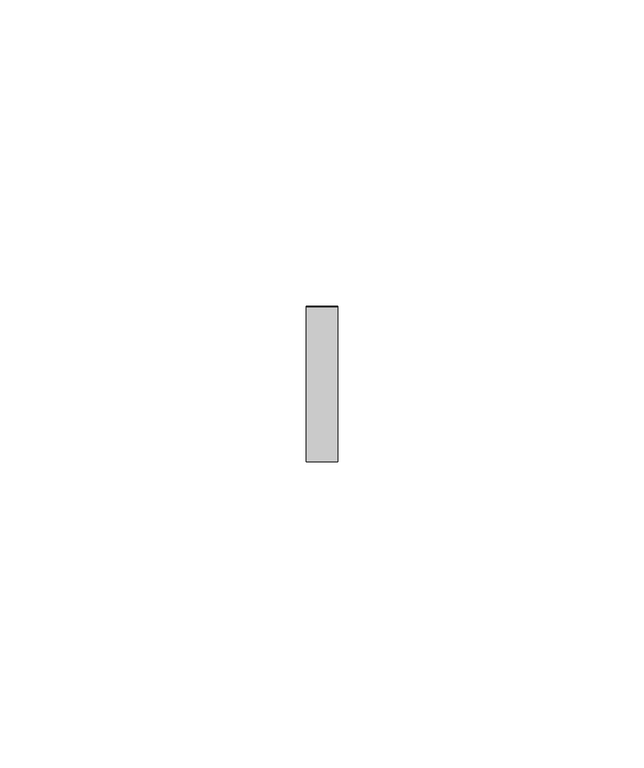
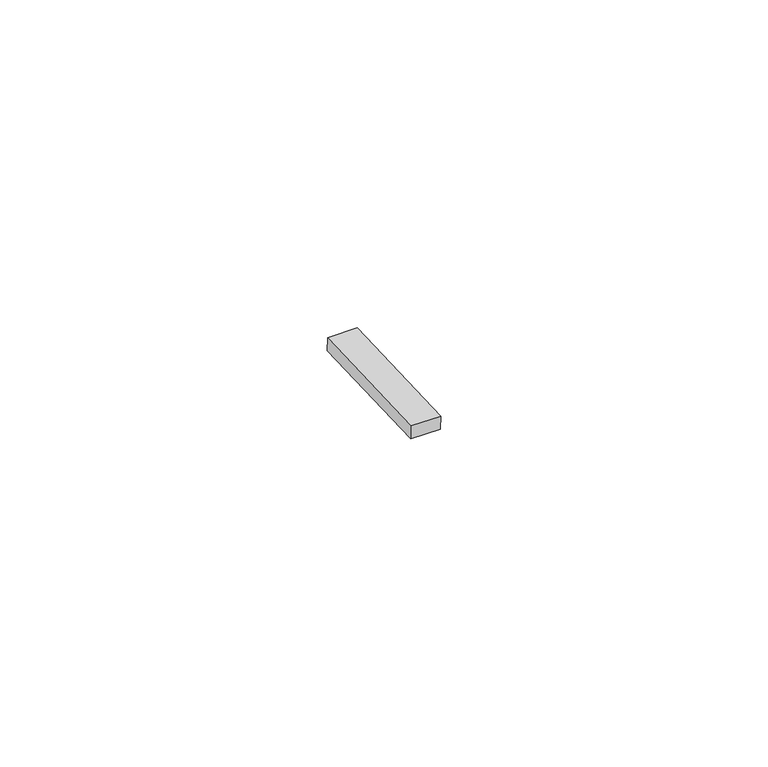
"""IFC4 building model written with IfcOpenShell, lengths in millimetres: proxy geometry, Inner panel:Inner panel:1:Inner panel:1 : Inner panel:Inner panel:300324:2:Inner panel:1:Inner panel:1 : Inner panel:Inner panel:300324:2 : Inner panel:Inner panel:1:Inner panel:1 : Inner panel:Inner panel:300324:300043:108 : Inner panel:Inner panel:1:Inner panel:1 : Inner panel:Inner panel:300324:2:Inner panel:1:Inner panel:1 : Inner panel:Inner panel:300324:2 : Inner panel:Inner panel:1:Inner panel:1 : Inner panel:Inner panel:300324:300043:308120."""

from ifc_helpers import new_model, si_unit, frame, origin, place, context, project, spatial, polyline, outline, extrude, source, transform, mapped, element, save


def generic_models_c30442cb(model_context):
    return source(origin(), model_context, "Body", "SweptSolid", [
        extrude(outline(polyline([(0.0, -25.4), (0.0, 0.0), (5.2138089, 0.0), (5.2138089, -25.4), (0.0, -25.4)])), frame((593530.195117, -576574.3073926, 4050.9976844), z_axis=(0.0, -0.041630544712223896, 0.9991330730923502), x_axis=(-1.0, 0.0, 0.0)), (0.0, 0.0, 1.0), 2.4763745),
    ])


if __name__ == "__main__":
    model = new_model("IFC4")
    model_context = context("Model", 3, world=origin())
    ifc_project = project(units=[si_unit("LENGTHUNIT", "METRE", prefix="MILLI")], contexts=[model_context])
    site = spatial("IfcSite", under=ifc_project)
    building = spatial("IfcBuilding", under=site)
    placement = place(None, origin())
    generic_models_shape = generic_models_c30442cb(model_context)
    element("IfcBuildingElementProxy", 1, Name="Inner panel:Inner panel:1:Inner panel:1 : Inner panel:Inner panel:300324:2:Inner panel:1:Inner panel:1 : Inner panel:Inner panel:300324:2 : Inner panel:Inner panel:1:Inner panel:1 : Inner panel:Inner panel:300324:300043:108 : Inner panel:Inner panel:1:Inner panel:1 : Inner panel:Inner panel:300324:2:Inner panel:1:Inner panel:1 : Inner panel:Inner panel:300324:2 : Inner panel:Inner panel:1:Inner panel:1 : Inner panel:Inner panel:300324:300043:308120", ObjectType="Inner panel:Inner panel:1:Inner panel:1 : Inner panel:Inner panel:300324:2:Inner panel:1:Inner panel:1 : Inner panel:Inner panel:300324:2 : Inner panel:Inner panel:1:Inner panel:1 : Inner panel:Inner panel:300324:300043:108 : Inner panel:Inner panel:1:Inner panel:1 : Inner panel:Inner panel:300324:2:Inner panel:1:Inner panel:1 : Inner panel:Inner panel:300324:2 : Inner panel:Inner panel:1:Inner panel:1 : Inner panel:Inner panel:300324:300043:308120", at=placement, inside=building, context=model_context, shape_type="MappedRepresentation", body=[
        mapped(generic_models_shape, transform((0.0, 0.0, 0.0), x_axis=(1.0, 0.0, 0.0), y_axis=(0.0, 1.0, 0.0), z_axis=(0.0, 0.0, 1.0))),
    ])
    save(model, "model.ifc")

# Revit data of these elements
# Type "Inner panel:Inner panel:1:Inner panel:1 : Inner panel:Inner panel:300324:2:Inner panel:1:Inner panel:1 : Inner panel:Inner panel:300324:2 : Inner panel:Inner panel:1:Inner panel:1 : Inner panel:Inner panel:300324:300043:108 : Inner panel:Inner panel:1:Inner panel:1 : Inner panel:Inner panel:300324:2:Inner panel:1:Inner panel:1 : Inner panel:Inner panel:300324:2 : Inner panel:Inner panel:1:Inner panel:1 : Inner panel:Inner panel:300324:300043:308120"
#   NameOverride = "Inner panel:Inner panel:1:Inner panel:1 : Inner panel:Inner panel:300324:2:Inner panel:1:Inner panel:1 : Inner panel:Inner panel:300324:2 : Inner panel:Inner panel:1:Inner panel:1 : Inner panel:Inner panel:300324:300043:308120"
#   ObjectTypeOverride = "Inner panel:1:Inner panel:1 : Inner panel:Inner panel:300324:2 : Inner panel:Inner panel:1:Inner panel:1 : Inner panel:Inner panel:300324:300043"
#   Reference = "Inner panel"
#   Tag = "308120"
# Element 1 (IfcBuildingElementProxy, "Inner panel:Inner panel:1:Inner panel:1 : Inner panel:Inner panel:300324:2:Inner panel:1:Inner panel:1 : Inner panel:Inner panel:300324:2 : Inner panel:Inner panel:1:Inner panel:1 : Inner panel:Inner panel:300324:300043:108 : Inner panel:Inner panel:1:Inner panel:1 : Inner panel:Inner panel:300324:2:Inner panel:1:Inner panel:1 : Inner panel:Inner panel:300324:2 : Inner panel:Inner panel:1:Inner panel:1 : Inner panel:Inner panel:300324:300043:308120")
#   Materials on its faces: "AT CLIP - 1\" WIDE NON ABSORBENT, WEATHER-RESISTANT NEOPRENE/EPDM/SBR FOAM"
# Materials
#   "AT CLIP - 1\" WIDE NON ABSORBENT, WEATHER-RESISTANT NEOPRENE/EPDM/SBR FOAM": class "Generic", colour RGB 85 85 85, transparency 0, Cost = 0
